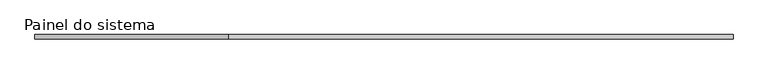
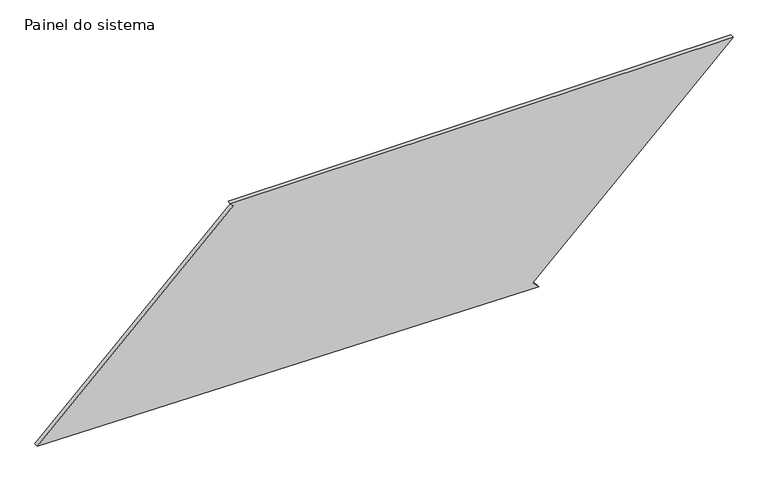
"""IFC4 building model written with IfcOpenShell, lengths in millimetres: plate geometry, Painel do sistema : Envidraçado."""

import ifcopenshell
import ifcopenshell.guid

model = None  # the IFC model being written
_history = None  # IfcOwnerHistory: only IFC2X3 demands one
_inside = {}  # id of a spatial element -> (the spatial element, [elements in it])
_under = {}  # id of a project, library or spatial element -> (it, [spatial elements below it])
_declared = {}  # id of a project -> (the project, [libraries it declares])
_typed = {}  # id of a type object -> (the type object, [elements of that type])
_made_of = {}  # id of a material, layer set ... -> (it, [elements and type objects made of it])


def new_model(schema):
    """Start an empty IFC model of exactly this schema.

    Asked for "IFC4X3", IfcOpenShell would pick the latest addendum, in which some entities
    have other attributes; the version numbers below select the first issue.
    IFC2X3 requires an IfcOwnerHistory on every rooted entity: one is made here for all.
    """
    global model, _history
    if schema == "IFC4X3":
        model = ifcopenshell.file(schema_version=(4, 3, 0, 0))
    else:
        model = ifcopenshell.file(schema=schema)
    _inside.clear()
    _under.clear()
    _declared.clear()
    _typed.clear()
    _made_of.clear()
    _history = None
    if model.schema == "IFC2X3":
        org = make("IfcOrganization", Name="unknown")
        user = make(
            "IfcPersonAndOrganization",
            ThePerson=make("IfcPerson", FamilyName="unknown"),
            TheOrganization=org,
        )
        app = make(
            "IfcApplication",
            ApplicationDeveloper=org,
            Version="unknown",
            ApplicationFullName="unknown",
            ApplicationIdentifier="unknown",
        )
        _history = make(
            "IfcOwnerHistory",
            OwningUser=user,
            OwningApplication=app,
            ChangeAction="ADDED",
            CreationDate=0,
        )
    return model


def make(cls, **values):
    """One entity of the class cls with the attributes given. An attribute that is None is left unset."""
    return model.create_entity(
        cls, **{name: value for name, value in values.items() if value is not None}
    )


def rooted(cls, **values):
    """An entity with a GlobalId (a new one), such as an element, a storey or a relation."""
    return make(cls, GlobalId=ifcopenshell.guid.new(), OwnerHistory=_history, **values)


def si_unit(unit_type, name, prefix=None):
    """IfcSIUnit, for example si_unit("LENGTHUNIT", "METRE", prefix="MILLI")."""
    return make("IfcSIUnit", UnitType=unit_type, Prefix=prefix, Name=name)


def assignment(units):
    """IfcUnitAssignment: the units of a project."""
    return None if units is None else make("IfcUnitAssignment", Units=units)


def point(xyz):
    """IfcCartesianPoint."""
    return None if xyz is None else make("IfcCartesianPoint", Coordinates=xyz)


def direction(xyz):
    """IfcDirection."""
    return None if xyz is None else make("IfcDirection", DirectionRatios=xyz)


def frame(location, z_axis=None, x_axis=None):
    """IfcAxis2Placement3D, a coordinate frame: its origin and axes. An axis left out is left unset."""
    return make(
        "IfcAxis2Placement3D",
        Location=point(location),
        Axis=direction(z_axis),
        RefDirection=direction(x_axis),
    )


def origin():
    """The frame at (0, 0, 0) with its axes left unset."""
    return frame((0.0, 0.0, 0.0))


def place(relative_to, where):
    """IfcLocalPlacement: puts the frame where relative to a parent placement (None: the world)."""
    return make(
        "IfcLocalPlacement", PlacementRelTo=relative_to, RelativePlacement=where
    )


def context(
    kind, dimensions, precision=None, world=None, true_north=None, identifier=None
):
    """IfcGeometricRepresentationContext, for example the 3D "Model" context."""
    return make(
        "IfcGeometricRepresentationContext",
        ContextIdentifier=identifier,
        ContextType=kind,
        CoordinateSpaceDimension=dimensions,
        Precision=precision,
        WorldCoordinateSystem=world,
        TrueNorth=true_north,
    )


def project(units=None, contexts=None):
    """IfcProject with its units and contexts."""
    return rooted(
        "IfcProject",
        Name="project",
        RepresentationContexts=contexts,
        UnitsInContext=assignment(units),
    )


def spatial(cls, under=None, at=None, **own):
    """A site, building, storey or space (cls), placed at a placement, below another one or the project."""
    s = rooted(cls, ObjectPlacement=at, **own)
    if under is not None:
        _under.setdefault(under.id(), (under, []))[1].append(s)
    return s


def polyline(points):
    """IfcPolyline through the points."""
    return make("IfcPolyline", Points=[point(p) for p in points])


def outline(outer, holes=None, kind="AREA"):
    """IfcArbitraryClosedProfileDef: a profile drawn as a closed curve; with holes, ...WithVoids."""
    if holes is None:
        return make("IfcArbitraryClosedProfileDef", ProfileType=kind, OuterCurve=outer)
    return make(
        "IfcArbitraryProfileDefWithVoids",
        ProfileType=kind,
        OuterCurve=outer,
        InnerCurves=holes,
    )


def extrude(swept, where, along, depth):
    """IfcExtrudedAreaSolid: the profile swept, set in the frame where, extruded along a direction by depth."""
    return make(
        "IfcExtrudedAreaSolid",
        SweptArea=swept,
        Position=where,
        ExtrudedDirection=direction(along),
        Depth=depth,
    )


def shape(context_of_items, identifier, shape_type, items):
    """IfcShapeRepresentation: the items that make up one representation, for example the "Body"."""
    return make(
        "IfcShapeRepresentation",
        ContextOfItems=context_of_items,
        RepresentationIdentifier=identifier,
        RepresentationType=shape_type,
        Items=items,
    )


def source(mapping_origin, context_of_items, identifier, shape_type, items):
    """IfcRepresentationMap: a shape defined once, which mapped items show again and again."""
    return make(
        "IfcRepresentationMap",
        MappingOrigin=mapping_origin,
        MappedRepresentation=shape(context_of_items, identifier, shape_type, items),
    )


def transform(
    local_origin,
    x_axis=None,
    y_axis=None,
    z_axis=None,
    scale=None,
    scale2=None,
    scale3=None,
    uniform=True,
):
    """IfcCartesianTransformationOperator3D, or its non-uniform kind. x_axis, y_axis, z_axis: its Axis1, 2, 3."""
    if uniform:
        return make(
            "IfcCartesianTransformationOperator3D",
            Axis1=direction(x_axis),
            Axis2=direction(y_axis),
            LocalOrigin=point(local_origin),
            Scale=scale,
            Axis3=direction(z_axis),
        )
    return make(
        "IfcCartesianTransformationOperator3DnonUniform",
        Axis1=direction(x_axis),
        Axis2=direction(y_axis),
        LocalOrigin=point(local_origin),
        Scale=scale,
        Axis3=direction(z_axis),
        Scale2=scale2,
        Scale3=scale3,
    )


def mapped(mapping_source, mapping_target):
    """IfcMappedItem: shows the shape of a source again, moved by a transform."""
    return make(
        "IfcMappedItem", MappingSource=mapping_source, MappingTarget=mapping_target
    )


def made_of(thing, what):
    """Note that an element or type object is made of a material, layer set ...; save() writes the relation."""
    if what is not None:
        _made_of.setdefault(what.id(), (what, []))[1].append(thing)
    return thing


def element(
    cls,
    number,
    at=None,
    inside=None,
    cuts=None,
    type_object=None,
    material=None,
    context=None,
    identifier="Body",
    shape_type=None,
    held_by="IfcProductDefinitionShape",
    body=None,
    shapes=None,
    **own,
):
    """One element of the class cls, such as IfcWall. Its Tag is "e" and its number.

    at: its placement. inside: the storey or other place that contains it. cuts: it is an
    opening in that element (IfcRelVoidsElement). A single representation is given by context,
    identifier, shape_type and body (its items); several are given by shapes. held_by: the class
    of the entity that holds the representations. save() writes the other relations.
    """
    e = rooted(cls, Tag="e%d" % number, ObjectPlacement=at, **own)
    if body is not None:
        shapes = [shape(context, identifier, shape_type, body)]
    if shapes is not None:
        e.Representation = make(held_by, Representations=shapes)
    if inside is not None:
        _inside.setdefault(inside.id(), (inside, []))[1].append(e)
    if cuts is not None:
        rooted(
            "IfcRelVoidsElement", RelatingBuildingElement=cuts, RelatedOpeningElement=e
        )
    if type_object is not None:
        _typed.setdefault(type_object.id(), (type_object, []))[1].append(e)
    return made_of(e, material)


def aggregate(whole, parts):
    """IfcRelAggregates: a whole, such as a stair, and the parts it consists of."""
    return rooted("IfcRelAggregates", RelatingObject=whole, RelatedObjects=parts)


def save(model, path):
    """Write the relations noted so far, then the file.

    IfcRelAggregates (storeys below a building ...), IfcRelContainedInSpatialStructure (elements
    in a storey), IfcRelDefinesByType, IfcRelAssociatesMaterial and IfcRelDeclares: one each for
    every whole, place, type object, material and project.
    """
    for whole, parts in _under.values():
        aggregate(whole, parts)
    for where, things in _inside.values():
        rooted(
            "IfcRelContainedInSpatialStructure",
            RelatedElements=things,
            RelatingStructure=where,
        )
    for kind, things in _typed.values():
        rooted("IfcRelDefinesByType", RelatedObjects=things, RelatingType=kind)
    for what, things in _made_of.values():
        rooted("IfcRelAssociatesMaterial", RelatedObjects=things, RelatingMaterial=what)
    for by, libraries in _declared.values():
        rooted("IfcRelDeclares", RelatingContext=by, RelatedDefinitions=libraries)
    model.write(path)


def painel_do_sistema_bdc71fc2(model_context):
    return source(origin(), model_context, "Body", "SweptSolid", [
        extrude(outline(polyline([(0.0, 926.2772659), (36.2928319, 891.8849652), (1180.8338574, 2099.6737491), (1180.8338574, -934.2251901), (1162.6874414, -917.0290398), (41.9737815, -2099.6737491), (0.0, 926.2772659)])), frame((0.0, 24.5, 0.0), z_axis=(0.0, 1.0, 0.0), x_axis=(0.0, 0.0, 1.0)), (0.0, 0.0, 1.0), 25.0),
    ])


if __name__ == "__main__":
    model = new_model("IFC4")
    model_context = context("Model", 3, world=origin())
    ifc_project = project(units=[si_unit("LENGTHUNIT", "METRE", prefix="MILLI")], contexts=[model_context])
    site = spatial("IfcSite", under=ifc_project)
    building = spatial("IfcBuilding", under=site)
    placement = place(None, origin())
    painel_do_sistema_shape = painel_do_sistema_bdc71fc2(model_context)
    element("IfcPlate", 1, ObjectType="Painel do sistema : Envidraçado", at=placement, inside=building, context=model_context, shape_type="MappedRepresentation", body=[
        mapped(painel_do_sistema_shape, transform((0.0, 0.0, 0.0), x_axis=(1.0, 0.0, 0.0), y_axis=(0.0, 1.0, 0.0), z_axis=(0.0, 0.0, 1.0))),
    ])
    save(model, "model.ifc")

# Revit data of these elements
# Type "Painel do sistema : Envidraçado"
#   Construction Type Id = "GSP4R"
#   Analytic Construction = "Vidraça única Pilkington 1/8 pol"
#   Visual Light Transmittance = 0.9
#   Solar Heat Gain Coefficient = 0.86
#   Heat Transfer Coefficient (U) = 6.7069 W/(m²·K)
# Element 1 (IfcPlate, "Painel do sistema : Envidraçado")
#   Materials on its faces: "Vidro"
# Materials
#   "Vidro": class "Vidro", colour RGB 0 128 192, transparency 0.9, Description = "Vidro de sílica", Cost = 0
